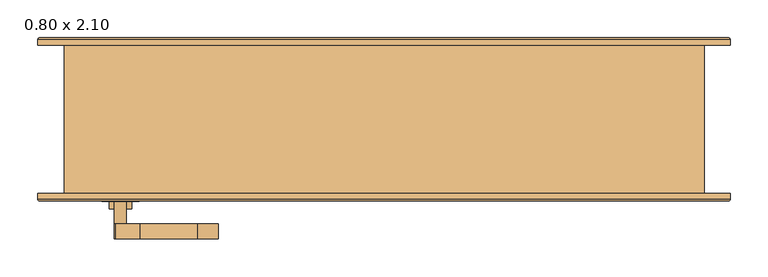
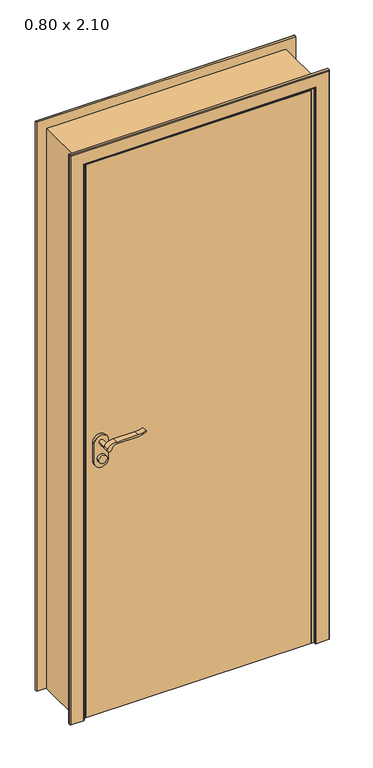
"""IFC4 building model written with IfcOpenShell, lengths in millimetres: door geometry, .CC_ND 300_PORTA SIMPLES DE ABRIR_COM EXTENSÃO : 0.80 x 2.10."""

from ifc_helpers import new_model, si_unit, point, frame, frame_2d, origin, origin_with_axes, place, context, project, spatial, polyline, circle_curve, ellipse_curve, trimmed, segment, composite_curve, outline, extrude, faceted_brep, source, transform, mapped, element, save
from ifc_brep_helpers import plane_surface, cylinder_surface, advanced_brep


def door_0_80_x_2_10_6c9b3ed6(model_context):
    return source(origin(), model_context, "Body", "SolidModel", [
        extrude(outline(composite_curve([segment(trimmed(circle_curve(frame_2d((964.5, -350.0)), 15.0), [point((964.5, -335.0))], [point((964.5, -365.0))], False, "CARTESIAN"), True, "CONTINUOUS"), segment(trimmed(circle_curve(frame_2d((964.5, -350.0)), 15.0), [point((964.5, -365.0))], [point((964.5, -335.0))], False, "CARTESIAN"), True, "CONTINUOUS")], self_intersect=False)), frame((0.0, -118.8, 0.0), z_axis=(0.0, 1.0, 0.0), x_axis=(0.0, 0.0, 1.0)), (0.0, 0.0, 1.0), 10.0),
        extrude(outline(composite_curve([segment(trimmed(circle_curve(frame_2d((964.5, -350.0)), 15.0), [point((964.5, -335.0))], [point((964.5, -365.0))], False, "CARTESIAN"), True, "CONTINUOUS"), segment(trimmed(circle_curve(frame_2d((964.5, -350.0)), 15.0), [point((964.5, -365.0))], [point((964.5, -335.0))], False, "CARTESIAN"), True, "CONTINUOUS")], self_intersect=False)), frame((0.0, -58.8, 0.0), z_axis=(0.0, 1.0, 0.0), x_axis=(0.0, 0.0, 1.0)), (0.0, 0.0, 1.0), 10.0),
        extrude(outline(composite_curve([segment(trimmed(circle_curve(frame_2d((1024.5, -350.0)), 8.0), [point((1029.1523287, -356.5081363))], [point((1024.5, -342.0))], False, "CARTESIAN"), True, "CONTINUOUS"), segment(trimmed(circle_curve(frame_2d((1019.3738613, -324.6138099)), 18.1261387), [point((1024.5, -342.0))], [point((1037.5, -324.6138099))], True, "CARTESIAN"), True, "CONTINUOUS"), segment(polyline([(1037.5, -324.6138099), (1037.5, -248.3564091)]), True, "CONTINUOUS"), segment(trimmed(circle_curve(frame_2d((1096.7709207, -251.9396612)), 59.3791355), [point((1037.5, -248.3564091))], [point((1046.7135558, -220.0))], False, "CARTESIAN"), True, "CONTINUOUS"), segment(polyline([(1046.7135558, -220.0), (1049.5, -220.0)]), True, "CONTINUOUS"), segment(trimmed(circle_curve(frame_2d((1127.7850638, -248.4227909)), 83.2850902), [point((1049.5, -220.0))], [point((1044.5, -248.3564091))], True, "CARTESIAN"), True, "CONTINUOUS"), segment(polyline([(1044.5, -248.3564091), (1044.5, -324.6325667)]), True, "CONTINUOUS"), segment(trimmed(circle_curve(frame_2d((1007.2555521, -326.3324871)), 37.2832219), [point((1044.5, -324.6325667))], [point((1029.1523287, -356.5081363))], False, "CARTESIAN"), True, "CONTINUOUS")], self_intersect=False)), frame((0.0, -158.8, 0.0), z_axis=(0.0, 1.0, 0.0), x_axis=(0.0, 0.0, 1.0)), (0.0, 0.0, 1.0), 20.0),
        extrude(outline(composite_curve([segment(trimmed(circle_curve(frame_2d((1019.3738682, -324.6138122)), 18.1261318), [point((1024.4999903, -342.0))], [point((1037.5, -324.6138122))], True, "CARTESIAN"), True, "CONTINUOUS"), segment(polyline([(1037.5, -324.6138122), (1037.5, -248.3564091)]), True, "CONTINUOUS"), segment(trimmed(circle_curve(frame_2d((1096.7709207, -251.9396612)), 59.3791355), [point((1037.5, -248.3564091))], [point((1046.7135558, -220.0))], False, "CARTESIAN"), True, "CONTINUOUS"), segment(polyline([(1046.7135558, -220.0), (1049.5, -220.0)]), True, "CONTINUOUS"), segment(trimmed(circle_curve(frame_2d((1127.7850638, -248.4227909)), 83.2850902), [point((1049.5, -220.0))], [point((1044.5, -248.3564091))], True, "CARTESIAN"), True, "CONTINUOUS"), segment(polyline([(1044.5, -248.3564091), (1044.5, -324.6325667)]), True, "CONTINUOUS"), segment(trimmed(circle_curve(frame_2d((1007.2555521, -326.3324871)), 37.2832219), [point((1044.5, -324.6325667))], [point((1029.1523287, -356.5081363))], False, "CARTESIAN"), True, "CONTINUOUS"), segment(trimmed(circle_curve(frame_2d((1024.5, -350.0)), 8.0), [point((1029.1523287, -356.5081363))], [point((1024.4999903, -342.0))], False, "CARTESIAN"), True, "CONTINUOUS")], self_intersect=False)), frame((0.0, -28.8, 0.0), z_axis=(0.0, 1.0, 0.0), x_axis=(0.0, 0.0, 1.0)), (0.0, 0.0, 1.0), 20.0),
        extrude(outline(composite_curve([segment(trimmed(circle_curve(frame_2d((1024.5, -350.0)), 8.0), [point((1024.5, -342.0))], [point((1024.5, -358.0))], False, "CARTESIAN"), True, "CONTINUOUS"), segment(trimmed(circle_curve(frame_2d((1024.5, -350.0)), 8.0), [point((1024.5, -358.0))], [point((1024.5, -342.0))], False, "CARTESIAN"), True, "CONTINUOUS")], self_intersect=False)), frame((0.0, -138.8, 0.0), z_axis=(0.0, 1.0, 0.0), x_axis=(0.0, 0.0, 1.0)), (0.0, 0.0, 1.0), 30.0),
        extrude(outline(composite_curve([segment(trimmed(circle_curve(frame_2d((1024.5, -350.0)), 8.0), [point((1024.5, -342.0))], [point((1024.5, -358.0))], False, "CARTESIAN"), True, "CONTINUOUS"), segment(trimmed(circle_curve(frame_2d((1024.5, -350.0)), 8.0), [point((1024.5, -358.0))], [point((1024.5, -342.0))], False, "CARTESIAN"), True, "CONTINUOUS")], self_intersect=False)), frame((0.0, -58.8, 0.0), z_axis=(0.0, 1.0, 0.0), x_axis=(0.0, 0.0, 1.0)), (0.0, 0.0, 1.0), 30.0),
        extrude(outline(composite_curve([segment(trimmed(circle_curve(frame_2d((954.5, -350.0)), 25.0), [point((954.5, -375.0))], [point((954.5, -325.0))], False, "CARTESIAN"), True, "CONTINUOUS"), segment(polyline([(954.5, -325.0), (1024.5, -325.0)]), True, "CONTINUOUS"), segment(trimmed(circle_curve(frame_2d((1024.5, -350.0)), 25.0), [point((1024.5, -325.0))], [point((1024.5, -375.0))], False, "CARTESIAN"), True, "CONTINUOUS"), segment(polyline([(1024.5, -375.0), (954.5, -375.0)]), True, "CONTINUOUS")], self_intersect=False)), frame((0.0, -108.8, 0.0), z_axis=(0.0, 1.0, 0.0), x_axis=(0.0, 0.0, 1.0)), (0.0, 0.0, 1.0), 10.0),
        extrude(outline(composite_curve([segment(trimmed(circle_curve(frame_2d((954.5, -350.0)), 25.0), [point((954.5, -375.0))], [point((954.5, -325.0))], False, "CARTESIAN"), True, "CONTINUOUS"), segment(polyline([(954.5, -325.0), (1024.5, -325.0)]), True, "CONTINUOUS"), segment(trimmed(circle_curve(frame_2d((1024.5, -350.0)), 25.0), [point((1024.5, -325.0))], [point((1024.5, -375.0))], False, "CARTESIAN"), True, "CONTINUOUS"), segment(polyline([(1024.5, -375.0), (954.5, -375.0)]), True, "CONTINUOUS")], self_intersect=False)), frame((0.0, -68.8, 0.0), z_axis=(0.0, 1.0, 0.0), x_axis=(0.0, 0.0, 1.0)), (0.0, 0.0, 1.0), 10.0),
        advanced_brep(
        [(-460.0, -98.8, 0.0), (-410.0, -98.8, 0.0), (-410.0, -105.8, 0.0), (-413.0, -108.8, 0.0), (-457.0, -108.8, 0.0), (-460.0, -105.8, 0.0), (-460.0, -98.8, 2135.0), (460.0, -98.8, 2135.0), (460.0, -98.8, 0.0), (410.0, -98.8, 0.0), (410.0, -98.8, 2085.0), (-410.0, -98.8, 2085.0), (-410.0, -105.8, 2085.0), (-413.0, -108.8, 2088.0), (413.0, -108.8, 2088.0), (413.0, -108.8, 0.0), (457.0, -108.8, 0.0), (457.0, -108.8, 2132.0), (-457.0, -108.8, 2132.0), (-460.0, -105.8, 2135.0), (460.0, -105.8, 2135.0), (460.0, -105.8, 0.0), (410.0, -105.8, 0.0), (410.0, -105.8, 2085.0)],
        [
            (0, 1),
            (1, 2),
            (2, 3, circle_curve(frame((-413.0, -105.8, 0.0), z_axis=(0.0, 0.0, -1.0), x_axis=(1.0, 0.0, 0.0)), 3.0)),
            (3, 4),
            (4, 5, circle_curve(frame((-457.0, -105.8, 0.0), z_axis=(0.0, 0.0, -1.0), x_axis=(1.0, 0.0, 0.0)), 3.0)),
            (5, 0),
            (0, 6),
            (6, 7),
            (7, 8),
            (8, 9),
            (9, 10),
            (10, 11),
            (11, 1),
            (11, 12),
            (12, 2),
            (12, 13, ellipse_curve(frame((-413.0, -105.8, 2088.0), z_axis=(-0.7071067811865475, 0.0, -0.7071067811865475), x_axis=(0.7071067811865474, 0.0, -0.7071067811865476)), 4.2426407, 3.0)),
            (13, 3),
            (13, 14),
            (14, 15),
            (15, 16),
            (16, 17),
            (17, 18),
            (18, 4),
            (18, 19, ellipse_curve(frame((-457.0, -105.8, 2132.0), z_axis=(-0.7071067811865475, 0.0, -0.7071067811865475), x_axis=(0.7071067811865474, 0.0, -0.7071067811865476)), 4.2426407, 3.0)),
            (19, 5),
            (19, 6),
            (7, 20),
            (20, 21),
            (21, 8),
            (21, 16, circle_curve(frame((457.0, -105.8, 0.0), z_axis=(0.0, 0.0, -1.0), x_axis=(-1.0, 0.0, 0.0)), 3.0)),
            (15, 22, circle_curve(frame((413.0, -105.8, 0.0), z_axis=(0.0, 0.0, -1.0), x_axis=(-1.0, 0.0, 0.0)), 3.0)),
            (22, 9),
            (23, 10),
            (22, 23),
            (14, 23, ellipse_curve(frame((413.0, -105.8, 2088.0), z_axis=(0.7071067811865475, 0.0, -0.7071067811865475), x_axis=(0.7071067811865474, 0.0, 0.7071067811865476)), 4.2426407, 3.0)),
            (20, 17, ellipse_curve(frame((457.0, -105.8, 2132.0), z_axis=(0.7071067811865475, 0.0, -0.7071067811865475), x_axis=(0.7071067811865474, 0.0, 0.7071067811865476)), 4.2426407, 3.0)),
            (23, 12),
            (19, 20),
        ],
        [
            plane_surface(frame((-410.0, -98.8, 0.0), z_axis=(0.0, 0.0, -1.0), x_axis=(0.0, 1.0, 0.0))),
            plane_surface(frame((-460.0, -98.8, 0.0), z_axis=(0.0, 1.0, 0.0), x_axis=(0.0, 0.0, 1.0))),
            plane_surface(frame((-410.0, -98.8, 0.0), z_axis=(1.0, 0.0, 0.0), x_axis=(0.0, 0.0, 1.0))),
            cylinder_surface(frame((-413.0, -105.8, 0.0), z_axis=(0.0, 0.0, -1.0), x_axis=(1.0, 0.0, 0.0)), 3.0),
            plane_surface(frame((-413.0, -108.8, 0.0), z_axis=(0.0, -1.0, 0.0), x_axis=(0.0, 0.0, 1.0))),
            cylinder_surface(frame((-457.0, -105.8, 0.0), z_axis=(0.0, 0.0, -1.0), x_axis=(1.0, 0.0, 0.0)), 3.0),
            plane_surface(frame((-460.0, -105.8, 0.0), z_axis=(-1.0, 0.0, 0.0), x_axis=(0.0, 0.0, 1.0))),
            plane_surface(frame((460.0, -105.8, 2135.0), z_axis=(1.0, 0.0, 0.0), x_axis=(0.0, 0.0, -1.0))),
            plane_surface(frame((410.0, -98.8, 0.0), z_axis=(0.0, 0.0, -1.0), x_axis=(0.0, 1.0, 0.0))),
            plane_surface(frame((410.0, -98.8, 2085.0), z_axis=(-1.0, 0.0, 0.0), x_axis=(0.0, 0.0, -1.0))),
            cylinder_surface(frame((413.0, -105.8, 2085.0), z_axis=(0.0, 0.0, 1.0), x_axis=(-1.0, 0.0, 0.0)), 3.0),
            cylinder_surface(frame((457.0, -105.8, 2085.0), z_axis=(0.0, 0.0, 1.0), x_axis=(-1.0, 0.0, 0.0)), 3.0),
            plane_surface(frame((-410.0, -98.8, 2085.0), z_axis=(0.0, 0.0, -1.0), x_axis=(1.0, 0.0, 0.0))),
            plane_surface(frame((-460.0, -105.8, 2135.0), z_axis=(0.0, 0.0, 1.0), x_axis=(1.0, 0.0, 0.0))),
            cylinder_surface(frame((-410.0, -105.8, 2088.0), z_axis=(-1.0, 0.0, 0.0), x_axis=(0.0, 0.0, -1.0)), 3.0),
            cylinder_surface(frame((-410.0, -105.8, 2132.0), z_axis=(-1.0, 0.0, 0.0), x_axis=(0.0, 0.0, -1.0)), 3.0),
        ],
        [
            (0, [[1, 2, 3, 4, 5, 6]]),
            (1, [[-1, 7, 8, 9, 10, 11, 12, 13]]),
            (2, [[-2, -13, 14, 15]]),
            (3, [[-3, -15, 16, 17]]),
            (4, [[-4, -17, 18, 19, 20, 21, 22, 23]]),
            (5, [[-5, -23, 24, 25]]),
            (6, [[-6, -25, 26, -7]]),
            (7, [[27, 28, 29, -9]]),
            (8, [[-29, 30, -20, 31, 32, -10]]),
            (9, [[33, -11, -32, 34]]),
            (10, [[35, -34, -31, -19]]),
            (11, [[36, -21, -30, -28]]),
            (12, [[-14, -12, -33, 37]]),
            (13, [[-26, 38, -27, -8]]),
            (14, [[-16, -37, -35, -18]]),
            (15, [[-24, -22, -36, -38]]),
        ],
    ),
        advanced_brep(
        [(460.0, 98.8, 0.0), (410.0, 98.8, 0.0), (410.0, 105.8157283, 0.0), (412.9842717, 108.8, 0.0), (457.0342217, 108.8, 0.0), (460.0, 105.8342217, 0.0), (460.0, 98.8, 2135.0), (-460.0, 98.8, 2135.0), (-460.0, 98.8, 0.0), (-410.0, 98.8, 0.0), (-410.0, 98.8, 2085.0), (410.0, 98.8, 2085.0), (410.0, 105.8157283, 2085.0), (412.9842717, 108.8, 2087.9842717), (-412.9842717, 108.8, 2087.9842717), (-412.9842717, 108.8, 0.0), (-457.0342217, 108.8, 0.0), (-457.0342217, 108.8, 2132.0342217), (457.0342217, 108.8, 2132.0342217), (460.0, 105.8342217, 2135.0), (-460.0, 105.8342217, 2135.0), (-460.0, 105.8342217, 0.0), (-410.0, 105.8157283, 0.0), (-410.0, 105.8157283, 2085.0)],
        [
            (0, 1),
            (1, 2),
            (2, 3, circle_curve(frame((412.9842717, 105.8157283, 0.0), z_axis=(0.0, 0.0, -1.0), x_axis=(1.0, 0.0, 0.0)), 2.9842717)),
            (3, 4),
            (4, 5, circle_curve(frame((457.0342217, 105.8342217, 0.0), z_axis=(0.0, 0.0, -1.0), x_axis=(1.0, 0.0, 0.0)), 2.9657783)),
            (5, 0),
            (0, 6),
            (6, 7),
            (7, 8),
            (8, 9),
            (9, 10),
            (10, 11),
            (11, 1),
            (11, 12),
            (12, 2),
            (12, 13, ellipse_curve(frame((412.9842717, 105.8157283, 2087.9842717), z_axis=(0.7071067811865475, 0.0, -0.7071067811865475), x_axis=(-0.7071067811865474, 0.0, -0.7071067811865476)), 4.2203975, 2.9842717)),
            (13, 3),
            (13, 14),
            (14, 15),
            (15, 16),
            (16, 17),
            (17, 18),
            (18, 4),
            (18, 19, ellipse_curve(frame((457.0342217, 105.8342217, 2132.0342217), z_axis=(0.7071067811865475, 0.0, -0.7071067811865475), x_axis=(-0.7071067811865474, 0.0, -0.7071067811865476)), 4.1942438, 2.9657783)),
            (19, 5),
            (19, 6),
            (7, 20),
            (20, 21),
            (21, 8),
            (21, 16, circle_curve(frame((-457.0342217, 105.8342217, 0.0), z_axis=(0.0, 0.0, -1.0), x_axis=(-1.0, 0.0, 0.0)), 2.9657783)),
            (15, 22, circle_curve(frame((-412.9842717, 105.8157283, 0.0), z_axis=(0.0, 0.0, -1.0), x_axis=(-1.0, 0.0, 0.0)), 2.9842717)),
            (22, 9),
            (23, 10),
            (22, 23),
            (14, 23, ellipse_curve(frame((-412.9842717, 105.8157283, 2087.9842717), z_axis=(-0.7071067811865475, 0.0, -0.7071067811865475), x_axis=(-0.7071067811865474, 0.0, 0.7071067811865476)), 4.2203975, 2.9842717)),
            (20, 17, ellipse_curve(frame((-457.0342217, 105.8342217, 2132.0342217), z_axis=(-0.7071067811865475, 0.0, -0.7071067811865475), x_axis=(-0.7071067811865474, 0.0, 0.7071067811865476)), 4.1942438, 2.9657783)),
            (23, 12),
            (19, 20),
        ],
        [
            plane_surface(frame((410.0, 98.8, 0.0), z_axis=(0.0, 0.0, -1.0), x_axis=(0.0, 1.0, 0.0))),
            plane_surface(frame((460.0, 98.8, 0.0), z_axis=(0.0, -1.0, 0.0), x_axis=(0.0, 0.0, 1.0))),
            plane_surface(frame((410.0, 98.8, 0.0), z_axis=(-1.0, 0.0, 0.0), x_axis=(0.0, 0.0, 1.0))),
            cylinder_surface(frame((412.9842717, 105.8157283, 0.0), z_axis=(0.0, 0.0, -1.0), x_axis=(1.0, 0.0, 0.0)), 2.9842717),
            plane_surface(frame((412.9842717, 108.8, 0.0), z_axis=(0.0, 1.0, 0.0), x_axis=(0.0, 0.0, 1.0))),
            cylinder_surface(frame((457.0342217, 105.8342217, 0.0), z_axis=(0.0, 0.0, -1.0), x_axis=(1.0, 0.0, 0.0)), 2.9657783),
            plane_surface(frame((460.0, 105.8342217, 0.0), z_axis=(1.0, 0.0, 0.0), x_axis=(0.0, 0.0, 1.0))),
            plane_surface(frame((-460.0, 105.8342217, 2135.0), z_axis=(-1.0, 0.0, 0.0), x_axis=(0.0, 0.0, -1.0))),
            plane_surface(frame((-410.0, 98.8, 0.0), z_axis=(0.0, 0.0, -1.0), x_axis=(0.0, 1.0, 0.0))),
            plane_surface(frame((-410.0, 98.8, 2085.0), z_axis=(1.0, 0.0, 0.0), x_axis=(0.0, 0.0, -1.0))),
            cylinder_surface(frame((-412.9842717, 105.8157283, 2085.0), z_axis=(0.0, 0.0, 1.0), x_axis=(-1.0, 0.0, 0.0)), 2.9842717),
            cylinder_surface(frame((-457.0342217, 105.8342217, 2085.0), z_axis=(0.0, 0.0, 1.0), x_axis=(-1.0, 0.0, 0.0)), 2.9657783),
            plane_surface(frame((410.0, 98.8, 2085.0), z_axis=(0.0, 0.0, -1.0), x_axis=(-1.0, 0.0, 0.0))),
            plane_surface(frame((460.0, 105.8342217, 2135.0), z_axis=(0.0, 0.0, 1.0), x_axis=(-1.0, 0.0, 0.0))),
            cylinder_surface(frame((410.0, 105.8157283, 2087.9842717), z_axis=(1.0, 0.0, 0.0), x_axis=(0.0, 0.0, 1.0)), 2.9842717),
            cylinder_surface(frame((410.0, 105.8342217, 2132.0342217), z_axis=(1.0, 0.0, 0.0), x_axis=(0.0, 0.0, 1.0)), 2.9657783),
        ],
        [
            (0, [[1, 2, 3, 4, 5, 6]]),
            (1, [[-1, 7, 8, 9, 10, 11, 12, 13]]),
            (2, [[-2, -13, 14, 15]]),
            (3, [[-3, -15, 16, 17]]),
            (4, [[-4, -17, 18, 19, 20, 21, 22, 23]]),
            (5, [[-5, -23, 24, 25]]),
            (6, [[-6, -25, 26, -7]]),
            (7, [[27, 28, 29, -9]]),
            (8, [[-29, 30, -20, 31, 32, -10]]),
            (9, [[33, -11, -32, 34]]),
            (10, [[35, -34, -31, -19]]),
            (11, [[36, -21, -30, -28]]),
            (12, [[-14, -12, -33, 37]]),
            (13, [[-26, 38, -27, -8]]),
            (14, [[-16, -37, -35, -18]]),
            (15, [[-24, -22, -36, -38]]),
        ],
    ),
        faceted_brep([(392.0, 98.8, 0.0), (425.0, 98.8, 0.0), (425.0, -98.8, 0.0), (400.0, -98.8, 0.0), (400.0, -68.8, 0.0), (392.0, -68.8, 0.0), (392.0, 98.8, 2067.0), (-392.0, 98.8, 2067.0), (-392.0, 98.8, 0.0), (-425.0, 98.8, 0.0), (-425.0, 98.8, 2100.0), (425.0, 98.8, 2100.0), (425.0, -98.8, 2100.0), (-425.0, -98.8, 2100.0), (-425.0, -98.8, 0.0), (-400.0, -98.8, 0.0), (-400.0, -98.8, 2075.0), (400.0, -98.8, 2075.0), (400.0, -68.8, 2075.0), (-400.0, -68.8, 2075.0), (-400.0, -68.8, 0.0), (-392.0, -68.8, 0.0), (-392.0, -68.8, 2067.0), (392.0, -68.8, 2067.0)], [[[0, 1, 2, 3, 4, 5]], [[1, 0, 6, 7, 8, 9, 10, 11]], [[2, 1, 11, 12]], [[3, 2, 12, 13, 14, 15, 16, 17]], [[4, 3, 17, 18]], [[5, 4, 18, 19, 20, 21, 22, 23]], [[0, 5, 23, 6]], [[7, 22, 21, 8]], [[8, 21, 20, 15, 14, 9]], [[13, 10, 9, 14]], [[19, 16, 15, 20]], [[12, 11, 10, 13]], [[18, 17, 16, 19]], [[6, 23, 22, 7]]]),
        extrude(outline(polyline([(-400.0, -68.8), (400.0, -68.8), (400.0, -98.8), (-400.0, -98.8), (-400.0, -68.8)])), origin_with_axes(), (0.0, 0.0, 1.0), 2075.0),
    ])


if __name__ == "__main__":
    model = new_model("IFC4")
    model_context = context("Model", 3, world=origin())
    ifc_project = project(units=[si_unit("LENGTHUNIT", "METRE", prefix="MILLI")], contexts=[model_context])
    site = spatial("IfcSite", under=ifc_project)
    building = spatial("IfcBuilding", under=site)
    placement = place(None, origin())
    door_0_80_x_2_10_shape = door_0_80_x_2_10_6c9b3ed6(model_context)
    element("IfcDoor", 1, ObjectType=".CC_ND 300_PORTA SIMPLES DE ABRIR_COM EXTENSÃO : 0.80 x 2.10", at=placement, inside=building, context=model_context, shape_type="MappedRepresentation", body=[
        mapped(door_0_80_x_2_10_shape, transform((0.0, 0.0, 0.0), x_axis=(1.0, 0.0, 0.0), y_axis=(0.0, 1.0, 0.0), z_axis=(0.0, 0.0, 1.0))),
    ])
    save(model, "model.ifc")

# Revit data of these elements
# Type ".CC_ND 300_PORTA SIMPLES DE ABRIR_COM EXTENSÃO : 0.80 x 2.10"
#   Type Mark = "153"
#   Rough Width = 0.85 m
#   Espessura moldura externa = 0.01 m
#   Espessura moldura interna = 0.01 m
#   Largura moldura = 0.05 m
#   Extensão acabamento exterior [instance default] = 0.00 m
#   Extensão acabamento interior [instance default] = 0.00 m
#   Espessura batente = 0.025 m
#   Thickness = 0.03 m
#   Altura batente = 2.085 m
#   Aux Arco [instance default] = 0.80 m
#   Rough Height = 2.125 m
#   Height = 2.10 m
#   Width = 0.80 m
#   Moldura interna [instance default] = yes
#   Moldura externa [instance default] = yes
#   Porta = .MADEIRA COM PINTURA ESMALTE BRANCO ACETINADO
#   Moldura = .MADEIRA COM PINTURA ESMALTE BRANCO ACETINADO
#   Maçaneta = .ALUMÍNIO
#   Batente = .MADEIRA COM PINTURA ESMALTE BRANCO ACETINADO
#   Function = (empty or 0)
#   Wall Closure = (empty or 0)
# Element 1 (IfcDoor, ".CC_ND 300_PORTA SIMPLES DE ABRIR_COM EXTENSÃO : 0.80 x 2.10")
#   Materials on its faces: ".MADEIRA COM PINTURA ESMALTE BRANCO ACETINADO", ".ALUMÍNIO"
# Materials
#   ".MADEIRA COM PINTURA ESMALTE BRANCO ACETINADO": class ".CC_MADEIRAS", colour RGB 240 240 240, transparency 0, Description = "Madeira com pintura esmalte branco acetinado.", Cost = 0
#   ".ALUMÍNIO": class "CC_METAIS", colour RGB 244 244 244, transparency 0, Description = "Material alumínio", Cost = 0
